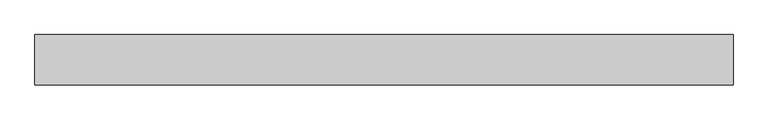
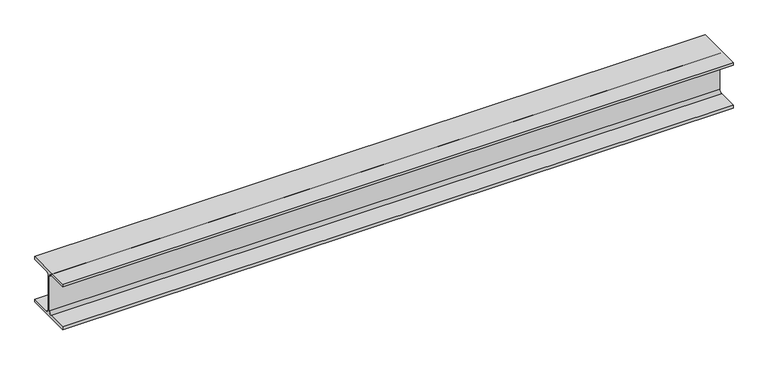
"""IFC4 building model written with IfcOpenShell, lengths in millimetres: beam geometry, 0912_Steel Framing_H-KSD3502 : H_SB_ASB_H-200x200x8x12."""

from ifc_helpers import new_model, si_unit, point, frame, frame_2d, origin, place, context, project, spatial, polyline, circle_curve, trimmed, segment, composite_curve, outline, extrude, source, transform, mapped, element, save


def beam_34493717(model_context):
    return source(origin(), model_context, "Body", "SweptSolid", [
        extrude(outline(composite_curve([segment(polyline([(100.0, -88.0), (100.0, -100.0), (-100.0, -100.0), (-100.0, -88.0), (-17.0, -88.0)]), True, "CONTINUOUS"), segment(trimmed(circle_curve(frame_2d((-17.0, -75.0)), 13.0), [point((-17.0, -88.0))], [point((-4.0, -75.0))], True, "CARTESIAN"), True, "CONTINUOUS"), segment(polyline([(-4.0, -75.0), (-4.0, 75.0)]), True, "CONTINUOUS"), segment(trimmed(circle_curve(frame_2d((-17.0, 75.0)), 13.0), [point((-4.0, 75.0))], [point((-17.0, 88.0))], True, "CARTESIAN"), True, "CONTINUOUS"), segment(polyline([(-17.0, 88.0), (-100.0, 88.0), (-100.0, 100.0), (100.0, 100.0), (100.0, 88.0), (17.0, 88.0)]), True, "CONTINUOUS"), segment(trimmed(circle_curve(frame_2d((17.0, 75.0)), 13.0), [point((17.0, 88.0))], [point((4.0, 75.0))], True, "CARTESIAN"), True, "CONTINUOUS"), segment(polyline([(4.0, 75.0), (4.0, -75.0)]), True, "CONTINUOUS"), segment(trimmed(circle_curve(frame_2d((17.0, -75.0)), 13.0), [point((4.0, -75.0))], [point((17.0, -88.0))], True, "CARTESIAN"), True, "CONTINUOUS"), segment(polyline([(17.0, -88.0), (100.0, -88.0)]), True, "CONTINUOUS")], self_intersect=False)), frame((-1399.4682263, 0.0, 0.0), z_axis=(1.0, 0.0, 0.0), x_axis=(0.0, 1.0, 0.0)), (0.0, 0.0, 1.0), 2781.1339085),
    ])


if __name__ == "__main__":
    model = new_model("IFC4")
    model_context = context("Model", 3, world=origin())
    ifc_project = project(units=[si_unit("LENGTHUNIT", "METRE", prefix="MILLI")], contexts=[model_context])
    site = spatial("IfcSite", under=ifc_project)
    building = spatial("IfcBuilding", under=site)
    placement = place(None, origin())
    beam_shape = beam_34493717(model_context)
    element("IfcBeam", 1, ObjectType="0912_Steel Framing_H-KSD3502 : H_SB_ASB_H-200x200x8x12", at=placement, inside=building, context=model_context, shape_type="MappedRepresentation", body=[
        mapped(beam_shape, transform((0.0, 0.0, 0.0), x_axis=(1.0, 0.0, 0.0), y_axis=(0.0, 1.0, 0.0), z_axis=(0.0, 0.0, 1.0))),
    ])
    save(model, "model.ifc")

# Revit data of these elements
# Type "0912_Steel Framing_H-KSD3502 : H_SB_ASB_H-200x200x8x12"
#   H_WM Code_1 = "S01AA002-00001 | Main Steel Structure Fabrication Work | Shelter/Building | Medium Steel - Standard (90KG/M>Weight≥30KG/M) | Material: (   )"
#   H_WM Code_2 = "S03AA028-00001 | Main Steel Structure Erection Work | Shelter/Building | Medium Steel (90KG/M>Weight≥30KG/M) | Material: (   )"
#   H_WM Code_3 = "S01AA010-00001 | Main Steel Structure Fabrication Work | Shelter/Building | Steel Painting/Coating | for Non-Fireproofed Steel Surface, Surface Preparation, Primer, Second & Final Coat | Material: (   )"
#   H_Q'ty Cal Type Tag = "SB-Q2"
#   Width = 20.0 cm
#   Web Thickness = 0.8 cm
#   Web Fillet = 1.3 cm
#   Warping Constant = 141000.0 cm⁶
#   W = 0
#   Torsional Moment of Inertia = 26.2485 cm⁴
#   Section Area = 63.53 cm²
#   Plastic Modulus weak axis = 244.0 cm³
#   Plastic Modulus strong axis = 525.0 cm³
#   Perimeter = 1.16 m²/m
#   Nominal Weight = 49.90 kgf/m
#   Moment of Inertia weak axis = 1600.00 cm⁴
#   Moment of Inertia strong axis = 4720.00 cm⁴
#   Height = 20.0 cm
#   Flange Thickness = 1.2 cm
#   Elastic Modulus weak axis = 160.0 cm³
#   Elastic Modulus strong axis = 472.0 cm³
#   Centroid Vertical = 10.0 cm
#   Centroid Horizontal = 10.0 cm
#   Ix = 47200000
#   Length [instance default] = 1.5240 m
#   Zx = 525000
#   b = 0.2000 m
#   h = 0.2000 m
#   r = 0.0130 m
#   s = 0.0080 m
#   t = 0.0120 m
#   A = 0.006353 m²
#   Structural Material [instance default] = Steel, 45-345
#   Assembly Code = ""
# Element 1 (IfcBeam, "0912_Steel Framing_H-KSD3502 : H_SB_ASB_H-200x200x8x12")
#   Structural Material = none
# Materials
#   "Steel, 45-345": class "Metal", colour RGB 189 187 185, transparency 0, Description = "Steel 345 MPa", Cost = 0
